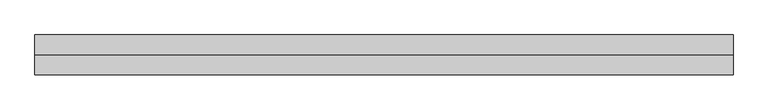
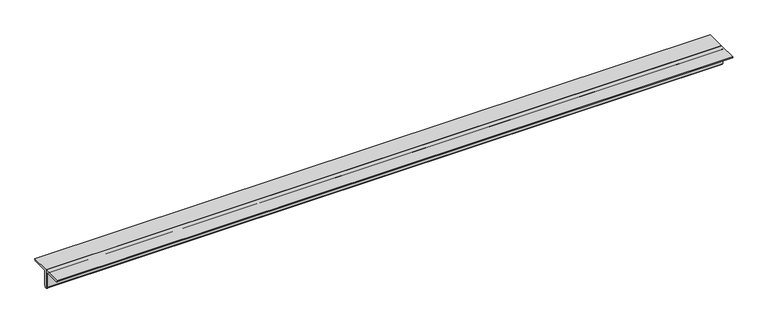
"""IFC4 building model written with IfcOpenShell, lengths in millimetres: member geometry, 0123_Steel Framing_2Ls-KSD3502 : H_SB_AR_S04_2Ls-130x130x12_VBR1."""

from ifc_helpers import new_model, si_unit, point, frame, frame_2d, origin, place, context, project, spatial, polyline, circle_curve, trimmed, segment, composite_curve, outline, extrude, source, transform, mapped, element, save


def member_5add8e11(model_context):
    return source(origin(), model_context, "Body", "SweptSolid", [
        extrude(outline(composite_curve([segment(polyline([(0.0, 36.4), (130.0, 36.4)]), True, "CONTINUOUS"), segment(trimmed(circle_curve(frame_2d((118.0, 36.4)), 12.0), [point((130.0, 36.4))], [point((118.0, 24.4))], False, "CARTESIAN"), True, "CONTINUOUS"), segment(polyline([(118.0, 24.4), (24.0, 24.4)]), True, "CONTINUOUS"), segment(trimmed(circle_curve(frame_2d((24.0, 12.4)), 12.0), [point((24.0, 24.4))], [point((12.0, 12.4))], True, "CARTESIAN"), True, "CONTINUOUS"), segment(polyline([(12.0, 12.4), (12.0, -81.6)]), True, "CONTINUOUS"), segment(trimmed(circle_curve(frame_2d((0.0, -81.6)), 12.0), [point((12.0, -81.6))], [point((0.0, -93.6))], False, "CARTESIAN"), True, "CONTINUOUS"), segment(polyline([(0.0, -93.6), (0.0, 36.4)]), True, "CONTINUOUS")], self_intersect=False)), frame((-2281.9000111, 0.0, 0.0), z_axis=(1.0, 0.0, 0.0), x_axis=(0.0, 1.0, 0.0)), (0.0, 0.0, 1.0), 4563.8000221),
        extrude(outline(composite_curve([segment(polyline([(0.0, 36.4), (0.0, -93.6)]), True, "CONTINUOUS"), segment(trimmed(circle_curve(frame_2d((0.0, -81.6)), 12.0), [point((0.0, -93.6))], [point((-12.0, -81.6))], False, "CARTESIAN"), True, "CONTINUOUS"), segment(polyline([(-12.0, -81.6), (-12.0, 12.4)]), True, "CONTINUOUS"), segment(trimmed(circle_curve(frame_2d((-24.0, 12.4)), 12.0), [point((-12.0, 12.4))], [point((-24.0, 24.4))], True, "CARTESIAN"), True, "CONTINUOUS"), segment(polyline([(-24.0, 24.4), (-118.0, 24.4)]), True, "CONTINUOUS"), segment(trimmed(circle_curve(frame_2d((-118.0, 36.4)), 12.0), [point((-118.0, 24.4))], [point((-130.0, 36.4))], False, "CARTESIAN"), True, "CONTINUOUS"), segment(polyline([(-130.0, 36.4), (0.0, 36.4)]), True, "CONTINUOUS")], self_intersect=False)), frame((-2281.9000111, 0.0, 0.0), z_axis=(1.0, 0.0, 0.0), x_axis=(0.0, 1.0, 0.0)), (0.0, 0.0, 1.0), 4563.8000221),
    ])


if __name__ == "__main__":
    model = new_model("IFC4")
    model_context = context("Model", 3, world=origin())
    ifc_project = project(units=[si_unit("LENGTHUNIT", "METRE", prefix="MILLI")], contexts=[model_context])
    site = spatial("IfcSite", under=ifc_project)
    building = spatial("IfcBuilding", under=site)
    placement = place(None, origin())
    member_shape = member_5add8e11(model_context)
    element("IfcMember", 1, ObjectType="0123_Steel Framing_2Ls-KSD3502 : H_SB_AR_S04_2Ls-130x130x12_VBR1", at=placement, inside=building, context=model_context, shape_type="MappedRepresentation", body=[
        mapped(member_shape, transform((0.0, 0.0, 0.0), x_axis=(1.0, 0.0, 0.0), y_axis=(0.0, 1.0, 0.0), z_axis=(0.0, 0.0, 1.0))),
    ])
    save(model, "model.ifc")

# Revit data of these elements
# Type "0123_Steel Framing_2Ls-KSD3502 : H_SB_AR_S04_2Ls-130x130x12_VBR1"
#   Assembly Code = "B10"
#   Legs = "SLBB"
#   W = 8.97
#   Perimeter = 1.04 m²/m
#   Nominal Weight = 46.80 kgf/m
#   Length [instance default] = 1000 mm
#   Space = 0 mm
#   b = 130 mm
#   d = 130 mm
#   t = 12 mm
#   y = 36.4 mm
#   A = 0.005952 m²
#   Structural Material [instance default] = Steel ASTM A36
# Element 1 (IfcMember, "0123_Steel Framing_2Ls-KSD3502 : H_SB_AR_S04_2Ls-130x130x12_VBR1")
#   Structural Material = Steel, 45-345
#   Materials on its faces: "Steel, 45-345"
# Materials
#   "Steel ASTM A36": class "Metal", colour RGB 199 199 199, transparency 0, Description = "Structural steel, ASTM A36 Grade B, mill finish", Cost = 0
#   "Steel, 45-345": class "Metal", colour RGB 189 187 185, transparency 0, Description = "Steel 345 MPa", Cost = 0
